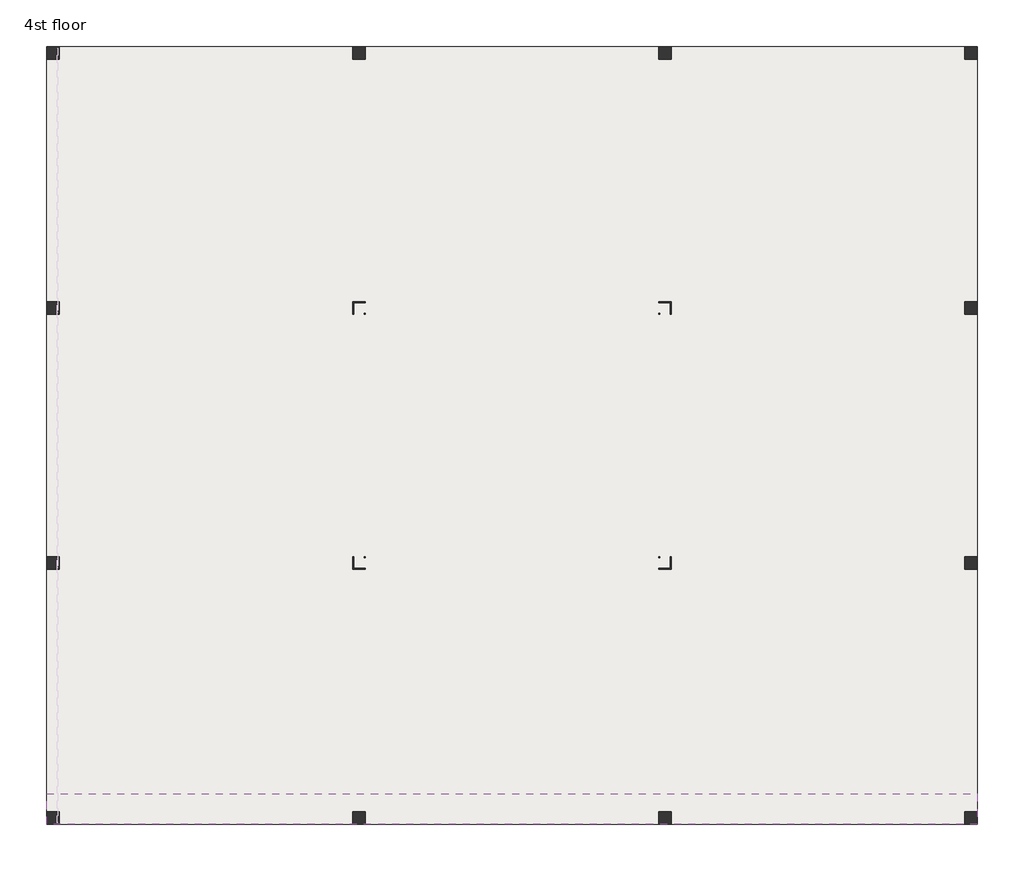
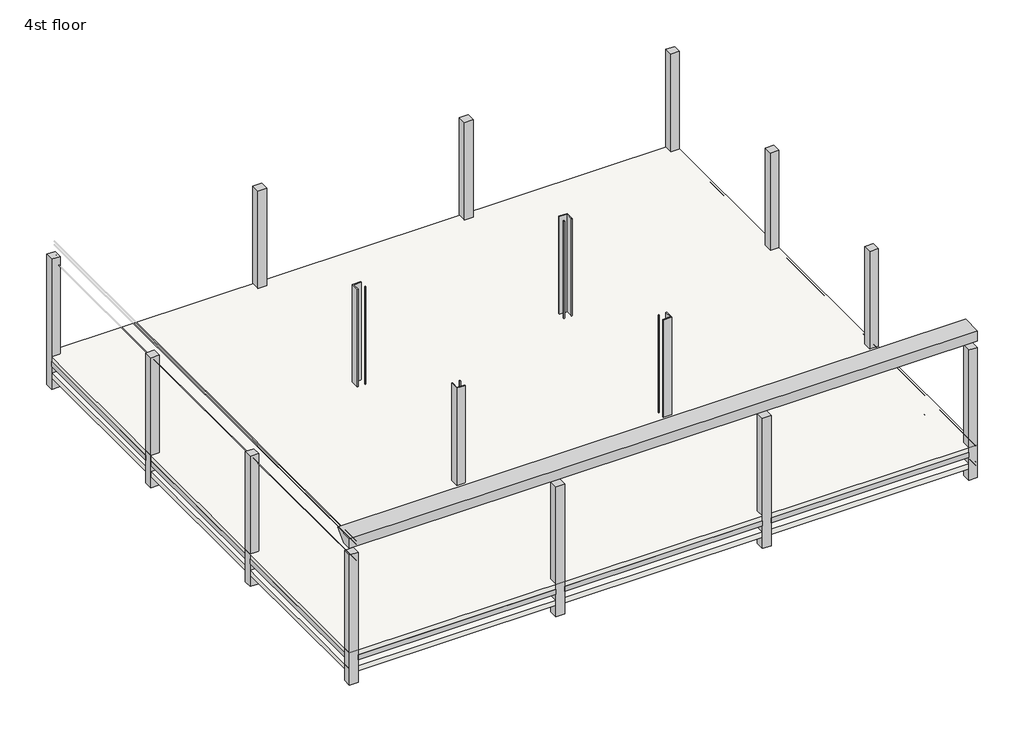
# One storey, part 1 of 2: 24 beams, 16 columns, 2 proxies, 2 slabs.
"""IFC4 building model written with IfcOpenShell, lengths in millimetres."""

import ifcopenshell
import ifcopenshell.guid

model = None  # the IFC model being written
_history = None  # IfcOwnerHistory: only IFC2X3 demands one
_inside = {}  # id of a spatial element -> (the spatial element, [elements in it])
_under = {}  # id of a project, library or spatial element -> (it, [spatial elements below it])
_declared = {}  # id of a project -> (the project, [libraries it declares])
_typed = {}  # id of a type object -> (the type object, [elements of that type])
_made_of = {}  # id of a material, layer set ... -> (it, [elements and type objects made of it])


def new_model(schema):
    """Start an empty IFC model of exactly this schema.

    Asked for "IFC4X3", IfcOpenShell would pick the latest addendum, in which some entities
    have other attributes; the version numbers below select the first issue.
    IFC2X3 requires an IfcOwnerHistory on every rooted entity: one is made here for all.
    """
    global model, _history
    if schema == "IFC4X3":
        model = ifcopenshell.file(schema_version=(4, 3, 0, 0))
    else:
        model = ifcopenshell.file(schema=schema)
    _inside.clear()
    _under.clear()
    _declared.clear()
    _typed.clear()
    _made_of.clear()
    _history = None
    if model.schema == "IFC2X3":
        org = make("IfcOrganization", Name="unknown")
        user = make(
            "IfcPersonAndOrganization",
            ThePerson=make("IfcPerson", FamilyName="unknown"),
            TheOrganization=org,
        )
        app = make(
            "IfcApplication",
            ApplicationDeveloper=org,
            Version="unknown",
            ApplicationFullName="unknown",
            ApplicationIdentifier="unknown",
        )
        _history = make(
            "IfcOwnerHistory",
            OwningUser=user,
            OwningApplication=app,
            ChangeAction="ADDED",
            CreationDate=0,
        )
    return model


def make(cls, **values):
    """One entity of the class cls with the attributes given. An attribute that is None is left unset."""
    return model.create_entity(
        cls, **{name: value for name, value in values.items() if value is not None}
    )


def rooted(cls, **values):
    """An entity with a GlobalId (a new one), such as an element, a storey or a relation."""
    return make(cls, GlobalId=ifcopenshell.guid.new(), OwnerHistory=_history, **values)


def si_unit(unit_type, name, prefix=None):
    """IfcSIUnit, for example si_unit("LENGTHUNIT", "METRE", prefix="MILLI")."""
    return make("IfcSIUnit", UnitType=unit_type, Prefix=prefix, Name=name)


def assignment(units):
    """IfcUnitAssignment: the units of a project."""
    return None if units is None else make("IfcUnitAssignment", Units=units)


def point(xyz):
    """IfcCartesianPoint."""
    return None if xyz is None else make("IfcCartesianPoint", Coordinates=xyz)


def direction(xyz):
    """IfcDirection."""
    return None if xyz is None else make("IfcDirection", DirectionRatios=xyz)


def frame(location, z_axis=None, x_axis=None):
    """IfcAxis2Placement3D, a coordinate frame: its origin and axes. An axis left out is left unset."""
    return make(
        "IfcAxis2Placement3D",
        Location=point(location),
        Axis=direction(z_axis),
        RefDirection=direction(x_axis),
    )


def origin():
    """The frame at (0, 0, 0) with its axes left unset."""
    return frame((0.0, 0.0, 0.0))


def place(relative_to, where):
    """IfcLocalPlacement: puts the frame where relative to a parent placement (None: the world)."""
    return make(
        "IfcLocalPlacement", PlacementRelTo=relative_to, RelativePlacement=where
    )


def context(
    kind, dimensions, precision=None, world=None, true_north=None, identifier=None
):
    """IfcGeometricRepresentationContext, for example the 3D "Model" context."""
    return make(
        "IfcGeometricRepresentationContext",
        ContextIdentifier=identifier,
        ContextType=kind,
        CoordinateSpaceDimension=dimensions,
        Precision=precision,
        WorldCoordinateSystem=world,
        TrueNorth=true_north,
    )


def project(units=None, contexts=None):
    """IfcProject with its units and contexts."""
    return rooted(
        "IfcProject",
        Name="project",
        RepresentationContexts=contexts,
        UnitsInContext=assignment(units),
    )


def spatial(cls, under=None, at=None, **own):
    """A site, building, storey or space (cls), placed at a placement, below another one or the project."""
    s = rooted(cls, ObjectPlacement=at, **own)
    if under is not None:
        _under.setdefault(under.id(), (under, []))[1].append(s)
    return s


def polyline(points):
    """IfcPolyline through the points."""
    return make("IfcPolyline", Points=[point(p) for p in points])


def outline(outer, holes=None, kind="AREA"):
    """IfcArbitraryClosedProfileDef: a profile drawn as a closed curve; with holes, ...WithVoids."""
    if holes is None:
        return make("IfcArbitraryClosedProfileDef", ProfileType=kind, OuterCurve=outer)
    return make(
        "IfcArbitraryProfileDefWithVoids",
        ProfileType=kind,
        OuterCurve=outer,
        InnerCurves=holes,
    )


def extrude(swept, where, along, depth):
    """IfcExtrudedAreaSolid: the profile swept, set in the frame where, extruded along a direction by depth."""
    return make(
        "IfcExtrudedAreaSolid",
        SweptArea=swept,
        Position=where,
        ExtrudedDirection=direction(along),
        Depth=depth,
    )


def faces_of(points, faces, orient=None, outer=None):
    """IfcFace entities. A face is a list of loops; a loop is a list of indices into points, from 0.

    orient and outer hold one flag for each loop. By default every Orientation is true, the
    first loop of a face is its IfcFaceOuterBound and the others are IfcFaceBound.
    """
    made = []
    for i, loops in enumerate(faces):
        bounds = []
        for j, loop in enumerate(loops):
            is_outer = j == 0 if outer is None else outer[i][j]
            bounds.append(
                make(
                    "IfcFaceOuterBound" if is_outer else "IfcFaceBound",
                    Bound=make("IfcPolyLoop", Polygon=[points[k] for k in loop]),
                    Orientation=True if orient is None else orient[i][j],
                )
            )
        made.append(make("IfcFace", Bounds=bounds))
    return made


def faceted_brep(points, faces, orient=None, outer=None, voids=None):
    """IfcFacetedBrep: a solid bounded by flat faces; with voids (closed shells), ...WithVoids."""
    shared = [point(p) for p in points]
    hull = make("IfcClosedShell", CfsFaces=faces_of(shared, faces, orient, outer))
    if voids is None:
        return make("IfcFacetedBrep", Outer=hull)
    return make(
        "IfcFacetedBrepWithVoids",
        Outer=hull,
        Voids=[
            make(cls, CfsFaces=faces_of(shared, fs, o, b)) for cls, fs, o, b in voids
        ],
    )


def shape(context_of_items, identifier, shape_type, items):
    """IfcShapeRepresentation: the items that make up one representation, for example the "Body"."""
    return make(
        "IfcShapeRepresentation",
        ContextOfItems=context_of_items,
        RepresentationIdentifier=identifier,
        RepresentationType=shape_type,
        Items=items,
    )


def made_of(thing, what):
    """Note that an element or type object is made of a material, layer set ...; save() writes the relation."""
    if what is not None:
        _made_of.setdefault(what.id(), (what, []))[1].append(thing)
    return thing


def element(
    cls,
    number,
    at=None,
    inside=None,
    cuts=None,
    type_object=None,
    material=None,
    context=None,
    identifier="Body",
    shape_type=None,
    held_by="IfcProductDefinitionShape",
    body=None,
    shapes=None,
    **own,
):
    """One element of the class cls, such as IfcWall. Its Tag is "e" and its number.

    at: its placement. inside: the storey or other place that contains it. cuts: it is an
    opening in that element (IfcRelVoidsElement). A single representation is given by context,
    identifier, shape_type and body (its items); several are given by shapes. held_by: the class
    of the entity that holds the representations. save() writes the other relations.
    """
    e = rooted(cls, Tag="e%d" % number, ObjectPlacement=at, **own)
    if body is not None:
        shapes = [shape(context, identifier, shape_type, body)]
    if shapes is not None:
        e.Representation = make(held_by, Representations=shapes)
    if inside is not None:
        _inside.setdefault(inside.id(), (inside, []))[1].append(e)
    if cuts is not None:
        rooted(
            "IfcRelVoidsElement", RelatingBuildingElement=cuts, RelatedOpeningElement=e
        )
    if type_object is not None:
        _typed.setdefault(type_object.id(), (type_object, []))[1].append(e)
    return made_of(e, material)


def aggregate(whole, parts):
    """IfcRelAggregates: a whole, such as a stair, and the parts it consists of."""
    return rooted("IfcRelAggregates", RelatingObject=whole, RelatedObjects=parts)


def save(model, path):
    """Write the relations noted so far, then the file.

    IfcRelAggregates (storeys below a building ...), IfcRelContainedInSpatialStructure (elements
    in a storey), IfcRelDefinesByType, IfcRelAssociatesMaterial and IfcRelDeclares: one each for
    every whole, place, type object, material and project.
    """
    for whole, parts in _under.values():
        aggregate(whole, parts)
    for where, things in _inside.values():
        rooted(
            "IfcRelContainedInSpatialStructure",
            RelatedElements=things,
            RelatingStructure=where,
        )
    for kind, things in _typed.values():
        rooted("IfcRelDefinesByType", RelatedObjects=things, RelatingType=kind)
    for what, things in _made_of.values():
        rooted("IfcRelAssociatesMaterial", RelatedObjects=things, RelatingMaterial=what)
    for by, libraries in _declared.values():
        rooted("IfcRelDeclares", RelatingContext=by, RelatedDefinitions=libraries)
    model.write(path)


model = new_model("IFC4")

# Units and contexts
model_context = context("Model", 3, world=origin())
ifc_project = project(units=[si_unit("LENGTHUNIT", "METRE", prefix="MILLI")], contexts=[model_context])

# Site, building, storey
site = spatial("IfcSite", under=ifc_project)
building = spatial("IfcBuilding", under=site)
storey = spatial("IfcBuildingStorey", under=building, Name="4st floor", Elevation=15500.0)

# Beams
placement = place(None, origin())
element("IfcBeam", 1, ObjectType="Concrete-Rectangular Beam : 250 x 300mm", at=placement, inside=storey, context=model_context, shape_type="SweptSolid", body=[
    extrude(outline(polyline([(-8833.7181639, -5693.2383613), (-8833.7181639, -5443.2383613), (-3083.7181639, -5443.2383613), (-3083.7181639, -5693.2383613), (-8833.7181639, -5693.2383613)])), frame((0.0, 0.0, 15200.0), z_axis=(0.0, 0.0, 1.0), x_axis=(1.0, 0.0, 0.0)), (0.0, 0.0, 1.0), 150.0),
])
element("IfcBeam", 2, ObjectType="Concrete-Rectangular Beam : 250 x 300mm", at=placement, inside=storey, context=model_context, shape_type="SweptSolid", body=[
    extrude(outline(polyline([(-2833.7181639, -5693.2383613), (-2833.7181639, -5443.2383613), (2916.2818361, -5443.2383613), (2916.2818361, -5693.2383613), (-2833.7181639, -5693.2383613)])), frame((0.0, 0.0, 15200.0), z_axis=(0.0, 0.0, 1.0), x_axis=(1.0, 0.0, 0.0)), (0.0, 0.0, 1.0), 150.0),
])
element("IfcBeam", 3, ObjectType="Concrete-Rectangular Beam : 250 x 300mm", at=placement, inside=storey, context=model_context, shape_type="SweptSolid", body=[
    extrude(outline(polyline([(3166.2818361, -5693.2383613), (3166.2818361, -5443.2383613), (8916.2818361, -5443.2383613), (8916.2818361, -5693.2383613), (3166.2818361, -5693.2383613)])), frame((0.0, 0.0, 15200.0), z_axis=(0.0, 0.0, 1.0), x_axis=(1.0, 0.0, 0.0)), (0.0, 0.0, 1.0), 150.0),
])
element("IfcBeam", 4, ObjectType="Concrete-Rectangular Beam : 250 x 300mm", at=placement, inside=storey, context=model_context, shape_type="SweptSolid", body=[
    extrude(outline(polyline([(-8833.7181639, -10443.2383613), (-9083.7181639, -10443.2383613), (-9083.7181639, -5693.2383613), (-8833.7181639, -5693.2383613), (-8833.7181639, -10443.2383613)])), frame((0.0, 0.0, 15200.0), z_axis=(0.0, 0.0, 1.0), x_axis=(1.0, 0.0, 0.0)), (0.0, 0.0, 1.0), 150.0),
])
element("IfcBeam", 5, ObjectType="Concrete-Rectangular Beam : 250 x 300mm", at=placement, inside=storey, context=model_context, shape_type="SweptSolid", body=[
    extrude(outline(polyline([(-8833.7181639, -15443.2383613), (-9083.7181639, -15443.2383613), (-9083.7181639, -10693.2383613), (-8833.7181639, -10693.2383613), (-8833.7181639, -15443.2383613)])), frame((0.0, 0.0, 15200.0), z_axis=(0.0, 0.0, 1.0), x_axis=(1.0, 0.0, 0.0)), (0.0, 0.0, 1.0), 150.0),
])
element("IfcBeam", 6, ObjectType="Concrete-Rectangular Beam : 250 x 300mm", at=placement, inside=storey, context=model_context, shape_type="SweptSolid", body=[
    extrude(outline(polyline([(-8833.7181639, -20443.2383613), (-9083.7181639, -20443.2383613), (-9083.7181639, -15693.2383613), (-8833.7181639, -15693.2383613), (-8833.7181639, -20443.2383613)])), frame((0.0, 0.0, 15200.0), z_axis=(0.0, 0.0, 1.0), x_axis=(1.0, 0.0, 0.0)), (0.0, 0.0, 1.0), 150.0),
])
element("IfcBeam", 7, ObjectType="Concrete-Rectangular Beam : 250 x 300mm", at=placement, inside=storey, context=model_context, shape_type="SweptSolid", body=[
    extrude(outline(polyline([(-2833.7181639, -10443.2383613), (-3083.7181639, -10443.2383613), (-3083.7181639, -5693.2383613), (-2833.7181639, -5693.2383613), (-2833.7181639, -10443.2383613)])), frame((0.0, 0.0, 15200.0), z_axis=(0.0, 0.0, 1.0), x_axis=(1.0, 0.0, 0.0)), (0.0, 0.0, 1.0), 150.0),
])
element("IfcBeam", 8, ObjectType="Concrete-Rectangular Beam : 250 x 300mm", at=placement, inside=storey, context=model_context, shape_type="SweptSolid", body=[
    extrude(outline(polyline([(-3083.7181639, -15443.2383613), (-3083.7181639, -10693.2383613), (-3058.7181639, -10693.2383613), (-3058.7181639, -15443.2383613), (-3083.7181639, -15443.2383613)])), frame((0.0, 0.0, 15200.0), z_axis=(0.0, 0.0, 1.0), x_axis=(1.0, 0.0, 0.0)), (0.0, 0.0, 1.0), 150.0),
    extrude(outline(polyline([(-2833.7181639, -10693.2383613), (-2833.7181639, -15443.2383613), (-2858.7181639, -15443.2383613), (-2858.7181639, -10693.2383613), (-2833.7181639, -10693.2383613)])), frame((0.0, 0.0, 15200.0), z_axis=(0.0, 0.0, 1.0), x_axis=(1.0, 0.0, 0.0)), (0.0, 0.0, 1.0), 150.0),
])
element("IfcBeam", 9, ObjectType="Concrete-Rectangular Beam : 250 x 300mm", at=placement, inside=storey, context=model_context, shape_type="SweptSolid", body=[
    extrude(outline(polyline([(-2833.7181639, -20443.2383613), (-3083.7181639, -20443.2383613), (-3083.7181639, -15693.2383613), (-2833.7181639, -15693.2383613), (-2833.7181639, -20443.2383613)])), frame((0.0, 0.0, 15200.0), z_axis=(0.0, 0.0, 1.0), x_axis=(1.0, 0.0, 0.0)), (0.0, 0.0, 1.0), 150.0),
])
element("IfcBeam", 10, ObjectType="Concrete-Rectangular Beam : 250 x 300mm", at=placement, inside=storey, context=model_context, shape_type="SweptSolid", body=[
    extrude(outline(polyline([(3166.2818361, -10443.2383613), (2916.2818361, -10443.2383613), (2916.2818361, -5693.2383613), (3166.2818361, -5693.2383613), (3166.2818361, -10443.2383613)])), frame((0.0, 0.0, 15200.0), z_axis=(0.0, 0.0, 1.0), x_axis=(1.0, 0.0, 0.0)), (0.0, 0.0, 1.0), 150.0),
])
element("IfcBeam", 11, ObjectType="Concrete-Rectangular Beam : 250 x 300mm", at=placement, inside=storey, context=model_context, shape_type="SweptSolid", body=[
    extrude(outline(polyline([(2916.2818361, -15443.2383613), (2916.2818361, -10693.2383613), (2941.2818361, -10693.2383613), (2941.2818361, -15443.2383613), (2916.2818361, -15443.2383613)])), frame((0.0, 0.0, 15200.0), z_axis=(0.0, 0.0, 1.0), x_axis=(1.0, 0.0, 0.0)), (0.0, 0.0, 1.0), 150.0),
    extrude(outline(polyline([(3166.2818361, -10693.2383613), (3166.2818361, -15443.2383613), (3141.2818361, -15443.2383613), (3141.2818361, -10693.2383613), (3166.2818361, -10693.2383613)])), frame((0.0, 0.0, 15200.0), z_axis=(0.0, 0.0, 1.0), x_axis=(1.0, 0.0, 0.0)), (0.0, 0.0, 1.0), 150.0),
])
element("IfcBeam", 12, ObjectType="Concrete-Rectangular Beam : 250 x 300mm", at=placement, inside=storey, context=model_context, shape_type="SweptSolid", body=[
    extrude(outline(polyline([(3166.2818361, -20443.2383613), (2916.2818361, -20443.2383613), (2916.2818361, -15693.2383613), (3166.2818361, -15693.2383613), (3166.2818361, -20443.2383613)])), frame((0.0, 0.0, 15200.0), z_axis=(0.0, 0.0, 1.0), x_axis=(1.0, 0.0, 0.0)), (0.0, 0.0, 1.0), 150.0),
])
element("IfcBeam", 13, ObjectType="Concrete-Rectangular Beam : 250 x 300mm", at=placement, inside=storey, context=model_context, shape_type="SweptSolid", body=[
    extrude(outline(polyline([(9166.2818361, -10443.2383613), (8916.2818361, -10443.2383613), (8916.2818361, -5693.2383613), (9166.2818361, -5693.2383613), (9166.2818361, -10443.2383613)])), frame((0.0, 0.0, 15200.0), z_axis=(0.0, 0.0, 1.0), x_axis=(1.0, 0.0, 0.0)), (0.0, 0.0, 1.0), 150.0),
])
element("IfcBeam", 14, ObjectType="Concrete-Rectangular Beam : 250 x 300mm", at=placement, inside=storey, context=model_context, shape_type="SweptSolid", body=[
    extrude(outline(polyline([(9166.2818361, -15443.2383613), (8916.2818361, -15443.2383613), (8916.2818361, -10693.2383613), (9166.2818361, -10693.2383613), (9166.2818361, -15443.2383613)])), frame((0.0, 0.0, 15200.0), z_axis=(0.0, 0.0, 1.0), x_axis=(1.0, 0.0, 0.0)), (0.0, 0.0, 1.0), 150.0),
])
element("IfcBeam", 15, ObjectType="Concrete-Rectangular Beam : 250 x 300mm", at=placement, inside=storey, context=model_context, shape_type="SweptSolid", body=[
    extrude(outline(polyline([(9166.2818361, -20443.2383613), (8916.2818361, -20443.2383613), (8916.2818361, -15693.2383613), (9166.2818361, -15693.2383613), (9166.2818361, -20443.2383613)])), frame((0.0, 0.0, 15200.0), z_axis=(0.0, 0.0, 1.0), x_axis=(1.0, 0.0, 0.0)), (0.0, 0.0, 1.0), 150.0),
])
element("IfcBeam", 16, ObjectType="Concrete-Rectangular Beam : 250 x 300mm", at=placement, inside=storey, context=model_context, shape_type="SweptSolid", body=[
    extrude(outline(polyline([(-8833.7181639, -20693.2383613), (-8833.7181639, -20443.2383613), (-3083.7181639, -20443.2383613), (-3083.7181639, -20693.2383613), (-8833.7181639, -20693.2383613)])), frame((0.0, 0.0, 15200.0), z_axis=(0.0, 0.0, 1.0), x_axis=(1.0, 0.0, 0.0)), (0.0, 0.0, 1.0), 150.0),
])
element("IfcBeam", 17, ObjectType="Concrete-Rectangular Beam : 250 x 300mm", at=placement, inside=storey, context=model_context, shape_type="SweptSolid", body=[
    extrude(outline(polyline([(-2833.7181639, -20693.2383613), (-2833.7181639, -20443.2383613), (2916.2818361, -20443.2383613), (2916.2818361, -20693.2383613), (-2833.7181639, -20693.2383613)])), frame((0.0, 0.0, 15200.0), z_axis=(0.0, 0.0, 1.0), x_axis=(1.0, 0.0, 0.0)), (0.0, 0.0, 1.0), 150.0),
])
element("IfcBeam", 18, ObjectType="Concrete-Rectangular Beam : 250 x 300mm", at=placement, inside=storey, context=model_context, shape_type="SweptSolid", body=[
    extrude(outline(polyline([(3166.2818361, -20693.2383613), (3166.2818361, -20443.2383613), (8916.2818361, -20443.2383613), (8916.2818361, -20693.2383613), (3166.2818361, -20693.2383613)])), frame((0.0, 0.0, 15200.0), z_axis=(0.0, 0.0, 1.0), x_axis=(1.0, 0.0, 0.0)), (0.0, 0.0, 1.0), 150.0),
])
element("IfcBeam", 19, ObjectType="Concrete-Rectangular Beam : 250 x 300mm", at=placement, inside=storey, context=model_context, shape_type="SweptSolid", body=[
    extrude(outline(polyline([(-8833.7181639, -15693.2383613), (-8833.7181639, -15443.2383613), (-3083.7181639, -15443.2383613), (-3083.7181639, -15693.2383613), (-8833.7181639, -15693.2383613)])), frame((0.0, 0.0, 15200.0), z_axis=(0.0, 0.0, 1.0), x_axis=(1.0, 0.0, 0.0)), (0.0, 0.0, 1.0), 150.0),
])
element("IfcBeam", 20, ObjectType="Concrete-Rectangular Beam : 250 x 300mm", at=placement, inside=storey, context=model_context, shape_type="SweptSolid", body=[
    extrude(outline(polyline([(2916.2818361, -15693.2383613), (-2833.7181639, -15693.2383613), (-2833.7181639, -15668.2383613), (2916.2818361, -15668.2383613), (2916.2818361, -15693.2383613)])), frame((0.0, 0.0, 15200.0), z_axis=(0.0, 0.0, 1.0), x_axis=(1.0, 0.0, 0.0)), (0.0, 0.0, 1.0), 150.0),
    extrude(outline(polyline([(-2833.7181639, -15443.2383613), (2916.2818361, -15443.2383613), (2916.2818361, -15468.2383613), (-2833.7181639, -15468.2383613), (-2833.7181639, -15443.2383613)])), frame((0.0, 0.0, 15200.0), z_axis=(0.0, 0.0, 1.0), x_axis=(1.0, 0.0, 0.0)), (0.0, 0.0, 1.0), 150.0),
])
element("IfcBeam", 21, ObjectType="Concrete-Rectangular Beam : 250 x 300mm", at=placement, inside=storey, context=model_context, shape_type="SweptSolid", body=[
    extrude(outline(polyline([(3166.2818361, -15693.2383613), (3166.2818361, -15443.2383613), (8916.2818361, -15443.2383613), (8916.2818361, -15693.2383613), (3166.2818361, -15693.2383613)])), frame((0.0, 0.0, 15200.0), z_axis=(0.0, 0.0, 1.0), x_axis=(1.0, 0.0, 0.0)), (0.0, 0.0, 1.0), 150.0),
])
element("IfcBeam", 22, ObjectType="Concrete-Rectangular Beam : 250 x 300mm", at=placement, inside=storey, context=model_context, shape_type="SweptSolid", body=[
    extrude(outline(polyline([(-8833.7181639, -10693.2383613), (-8833.7181639, -10443.2383613), (-3083.7181639, -10443.2383613), (-3083.7181639, -10693.2383613), (-8833.7181639, -10693.2383613)])), frame((0.0, 0.0, 15200.0), z_axis=(0.0, 0.0, 1.0), x_axis=(1.0, 0.0, 0.0)), (0.0, 0.0, 1.0), 150.0),
])
element("IfcBeam", 23, ObjectType="Concrete-Rectangular Beam : 250 x 300mm", at=placement, inside=storey, context=model_context, shape_type="SweptSolid", body=[
    extrude(outline(polyline([(2916.2818361, -10693.2383613), (-2833.7181639, -10693.2383613), (-2833.7181639, -10668.2383613), (2916.2818361, -10668.2383613), (2916.2818361, -10693.2383613)])), frame((0.0, 0.0, 15200.0), z_axis=(0.0, 0.0, 1.0), x_axis=(1.0, 0.0, 0.0)), (0.0, 0.0, 1.0), 150.0),
    extrude(outline(polyline([(-2833.7181639, -10443.2383613), (2916.2818361, -10443.2383613), (2916.2818361, -10468.2383613), (-2833.7181639, -10468.2383613), (-2833.7181639, -10443.2383613)])), frame((0.0, 0.0, 15200.0), z_axis=(0.0, 0.0, 1.0), x_axis=(1.0, 0.0, 0.0)), (0.0, 0.0, 1.0), 150.0),
])
element("IfcBeam", 24, ObjectType="Concrete-Rectangular Beam : 250 x 300mm", at=placement, inside=storey, context=model_context, shape_type="SweptSolid", body=[
    extrude(outline(polyline([(3166.2818361, -10693.2383613), (3166.2818361, -10443.2383613), (8916.2818361, -10443.2383613), (8916.2818361, -10693.2383613), (3166.2818361, -10693.2383613)])), frame((0.0, 0.0, 15200.0), z_axis=(0.0, 0.0, 1.0), x_axis=(1.0, 0.0, 0.0)), (0.0, 0.0, 1.0), 150.0),
])

# Proxies
element("IfcBuildingElementProxy", 25, Name="Slab Edge", ObjectType="Slab Edge", at=placement, inside=storey, context=model_context, shape_type="SweptSolid", body=[
    extrude(outline(polyline([(-20693.2383613, 18700.0), (-20693.2383613, 19000.0), (-20093.2383613, 19000.0), (-20393.2383613, 18700.0), (-20693.2383613, 18700.0)])), frame((-9083.7181639, 0.0, 0.0), z_axis=(1.0, 0.0, 0.0), x_axis=(0.0, 1.0, 0.0)), (0.0, 0.0, 1.0), 18250.0),
])
element("IfcBuildingElementProxy", 26, Name="Slab Edge", ObjectType="Slab Edge", at=placement, inside=storey, context=model_context, shape_type="SweptSolid", body=[
    extrude(outline(polyline([(-20693.2383613, 18700.0), (-20693.2383613, 19000.0), (-20093.2383613, 19000.0), (-20393.2383613, 18700.0), (-20693.2383613, 18700.0)])), frame((-9083.7181639, 0.0, 0.0), z_axis=(1.0, 0.0, 0.0), x_axis=(0.0, 1.0, 0.0)), (0.0, 0.0, 1.0), 18250.0),
])

# Columns
element("IfcColumn", 27, ObjectType="Concrete-Rectangular-Column : 250x250 mm", at=placement, inside=storey, context=model_context, shape_type="Brep", body=[
    faceted_brep([(-8833.7181639, -20443.2383613, 18500.0), (-9083.7181639, -20443.2383613, 18500.0), (-9083.7181639, -20693.2383613, 18500.0), (-8833.7181639, -20693.2383613, 18500.0), (-8833.7181639, -20443.2383613, 14500.0), (-8833.7181639, -20693.2383613, 14500.0), (-9083.7181639, -20693.2383613, 14500.0), (-9083.7181639, -20443.2383613, 14500.0), (-8833.7181639, -20443.2383613, 14850.0), (-8833.7181639, -20443.2383613, 14700.0), (-9083.7181639, -20443.2383613, 14700.0), (-9083.7181639, -20443.2383613, 14850.0), (-8833.7181639, -20693.2383613, 14700.0), (-8833.7181639, -20693.2383613, 14850.0)], [[[0, 1, 2, 3]], [[4, 5, 6, 7]], [[1, 0, 8, 9, 4, 7, 10, 11]], [[2, 1, 11, 10, 7, 6]], [[3, 2, 6, 5, 12, 13]], [[0, 3, 13, 12, 5, 4, 9, 8]]]),
])
element("IfcColumn", 28, ObjectType="Concrete-Rectangular-Column : 250x250 mm", at=placement, inside=storey, context=model_context, shape_type="Brep", body=[
    faceted_brep([(-8833.7181639, -15443.2383613, 18500.0), (-9083.7181639, -15443.2383613, 18500.0), (-9083.7181639, -15693.2383613, 18500.0), (-8833.7181639, -15693.2383613, 18500.0), (-8833.7181639, -15443.2383613, 14500.0), (-8833.7181639, -15693.2383613, 14500.0), (-9083.7181639, -15693.2383613, 14500.0), (-9083.7181639, -15443.2383613, 14500.0), (-8833.7181639, -15443.2383613, 14850.0), (-8833.7181639, -15443.2383613, 14700.0), (-9083.7181639, -15443.2383613, 14700.0), (-9083.7181639, -15443.2383613, 14850.0), (-9083.7181639, -15693.2383613, 14700.0), (-9083.7181639, -15693.2383613, 14850.0), (-8833.7181639, -15693.2383613, 14700.0), (-8833.7181639, -15693.2383613, 14850.0)], [[[0, 1, 2, 3]], [[4, 5, 6, 7]], [[1, 0, 8, 9, 4, 7, 10, 11]], [[2, 1, 11, 10, 7, 6, 12, 13]], [[3, 2, 13, 12, 6, 5, 14, 15]], [[0, 3, 15, 14, 5, 4, 9, 8]]]),
])
element("IfcColumn", 29, ObjectType="Concrete-Rectangular-Column : 250x250 mm", at=placement, inside=storey, context=model_context, shape_type="Brep", body=[
    faceted_brep([(-8833.7181639, -10443.2383613, 18500.0), (-9083.7181639, -10443.2383613, 18500.0), (-9083.7181639, -10693.2383613, 18500.0), (-8833.7181639, -10693.2383613, 18500.0), (-8833.7181639, -10443.2383613, 14500.0), (-8833.7181639, -10693.2383613, 14500.0), (-9083.7181639, -10693.2383613, 14500.0), (-9083.7181639, -10443.2383613, 14500.0), (-8833.7181639, -10443.2383613, 14850.0), (-8833.7181639, -10443.2383613, 14700.0), (-9083.7181639, -10443.2383613, 14700.0), (-9083.7181639, -10443.2383613, 14850.0), (-9083.7181639, -10693.2383613, 14700.0), (-9083.7181639, -10693.2383613, 14850.0), (-8833.7181639, -10693.2383613, 14700.0), (-8833.7181639, -10693.2383613, 14850.0)], [[[0, 1, 2, 3]], [[4, 5, 6, 7]], [[1, 0, 8, 9, 4, 7, 10, 11]], [[2, 1, 11, 10, 7, 6, 12, 13]], [[3, 2, 13, 12, 6, 5, 14, 15]], [[0, 3, 15, 14, 5, 4, 9, 8]]]),
])
element("IfcColumn", 30, ObjectType="Concrete-Rectangular-Column : 250x250 mm", at=placement, inside=storey, context=model_context, shape_type="Brep", body=[
    faceted_brep([(-8833.7181639, -5443.2383613, 18500.0), (-9083.7181639, -5443.2383613, 18500.0), (-9083.7181639, -5693.2383613, 18500.0), (-8833.7181639, -5693.2383613, 18500.0), (-8833.7181639, -5443.2383613, 14500.0), (-8833.7181639, -5693.2383613, 14500.0), (-9083.7181639, -5693.2383613, 14500.0), (-9083.7181639, -5443.2383613, 14500.0), (-8833.7181639, -5443.2383613, 14850.0), (-8833.7181639, -5443.2383613, 14700.0), (-9083.7181639, -5693.2383613, 14700.0), (-9083.7181639, -5693.2383613, 14850.0), (-8833.7181639, -5693.2383613, 14700.0), (-8833.7181639, -5693.2383613, 14850.0)], [[[0, 1, 2, 3]], [[4, 5, 6, 7]], [[1, 0, 8, 9, 4, 7]], [[2, 1, 7, 6, 10, 11]], [[3, 2, 11, 10, 6, 5, 12, 13]], [[0, 3, 13, 12, 5, 4, 9, 8]]]),
])
element("IfcColumn", 31, ObjectType="Concrete-Rectangular-Column : 250x250 mm", at=placement, inside=storey, context=model_context, shape_type="Brep", body=[
    faceted_brep([(-2833.7181639, -20443.2383613, 18500.0), (-3083.7181639, -20443.2383613, 18500.0), (-3083.7181639, -20693.2383613, 18500.0), (-2833.7181639, -20693.2383613, 18500.0), (-2833.7181639, -20443.2383613, 14500.0), (-2833.7181639, -20693.2383613, 14500.0), (-3083.7181639, -20693.2383613, 14500.0), (-3083.7181639, -20443.2383613, 14500.0), (-2833.7181639, -20443.2383613, 14850.0), (-2833.7181639, -20443.2383613, 14700.0), (-3083.7181639, -20443.2383613, 14700.0), (-3083.7181639, -20443.2383613, 14850.0), (-3083.7181639, -20693.2383613, 14700.0), (-3083.7181639, -20693.2383613, 14850.0), (-2833.7181639, -20693.2383613, 14700.0), (-2833.7181639, -20693.2383613, 14850.0)], [[[0, 1, 2, 3]], [[4, 5, 6, 7]], [[1, 0, 8, 9, 4, 7, 10, 11]], [[2, 1, 11, 10, 7, 6, 12, 13]], [[3, 2, 13, 12, 6, 5, 14, 15]], [[0, 3, 15, 14, 5, 4, 9, 8]]]),
])
element("IfcColumn", 32, ObjectType="Concrete-Rectangular-Column : 250x250 mm", at=placement, inside=storey, context=model_context, shape_type="Brep", body=[
    faceted_brep([(-2833.7181639, -15468.2383613, 18500.0), (-2833.7181639, -15443.2383613, 18500.0), (-2858.7181639, -15443.2383613, 18500.0), (-2858.7181639, -15468.2383613, 18500.0), (-2833.7181639, -15443.2383613, 14500.0), (-2833.7181639, -15468.2383613, 14500.0), (-2858.7181639, -15468.2383613, 14500.0), (-2858.7181639, -15443.2383613, 14500.0), (-2833.7181639, -15443.2383613, 14850.0), (-2833.7181639, -15443.2383613, 14700.0), (-2858.7181639, -15443.2383613, 14700.0), (-2858.7181639, -15443.2383613, 14850.0), (-2833.7181639, -15468.2383613, 14850.0), (-2833.7181639, -15468.2383613, 14700.0)], [[[0, 1, 2, 3]], [[4, 5, 6, 7]], [[1, 8, 9, 4, 7, 10, 11, 2]], [[4, 9, 8, 1, 0, 12, 13, 5]], [[5, 13, 12, 0, 3, 6]], [[3, 2, 11, 10, 7, 6]]]),
    faceted_brep([(-3083.7181639, -15693.2383613, 18500.0), (-3083.7181639, -15443.2383613, 18500.0), (-3083.7181639, -15443.2383613, 14850.0), (-3083.7181639, -15443.2383613, 14700.0), (-3083.7181639, -15443.2383613, 14500.0), (-3083.7181639, -15693.2383613, 14500.0), (-3083.7181639, -15693.2383613, 14700.0), (-3083.7181639, -15693.2383613, 14850.0), (-2833.7181639, -15693.2383613, 18500.0), (-2833.7181639, -15693.2383613, 14500.0), (-2833.7181639, -15693.2383613, 14700.0), (-2833.7181639, -15693.2383613, 14850.0), (-3058.7181639, -15668.2383613, 14500.0), (-3058.7181639, -15668.2383613, 18500.0), (-2833.7181639, -15668.2383613, 18500.0), (-2833.7181639, -15668.2383613, 14850.0), (-2833.7181639, -15668.2383613, 14700.0), (-2833.7181639, -15668.2383613, 14500.0), (-3058.7181639, -15443.2383613, 14500.0), (-3058.7181639, -15443.2383613, 14700.0), (-3058.7181639, -15443.2383613, 14850.0), (-3058.7181639, -15443.2383613, 18500.0)], [[[0, 1, 2, 3, 4, 5, 6, 7]], [[8, 0, 7, 6, 5, 9, 10, 11]], [[12, 13, 14, 15, 16, 17]], [[13, 12, 18, 19, 20, 21]], [[8, 11, 10, 9, 17, 16, 15, 14]], [[1, 0, 8, 14, 13, 21]], [[9, 5, 4, 18, 12, 17]], [[4, 3, 2, 1, 21, 20, 19, 18]]]),
])
element("IfcColumn", 33, ObjectType="Concrete-Rectangular-Column : 250x250 mm", at=placement, inside=storey, context=model_context, shape_type="Brep", body=[
    faceted_brep([(-2833.7181639, -10443.2383613, 18500.0), (-3083.7181639, -10443.2383613, 18500.0), (-3083.7181639, -10693.2383613, 18500.0), (-3058.7181639, -10693.2383613, 18500.0), (-3058.7181639, -10468.2383613, 18500.0), (-2833.7181639, -10468.2383613, 18500.0), (-3083.7181639, -10693.2383613, 14500.0), (-3083.7181639, -10443.2383613, 14500.0), (-2833.7181639, -10443.2383613, 14500.0), (-2833.7181639, -10468.2383613, 14500.0), (-3058.7181639, -10468.2383613, 14500.0), (-3058.7181639, -10693.2383613, 14500.0), (-2833.7181639, -10443.2383613, 14850.0), (-2833.7181639, -10443.2383613, 14700.0), (-3083.7181639, -10443.2383613, 14700.0), (-3083.7181639, -10443.2383613, 14850.0), (-3083.7181639, -10693.2383613, 14700.0), (-3083.7181639, -10693.2383613, 14850.0), (-3058.7181639, -10693.2383613, 14700.0), (-3058.7181639, -10693.2383613, 14850.0), (-2833.7181639, -10468.2383613, 14850.0), (-2833.7181639, -10468.2383613, 14700.0)], [[[0, 1, 2, 3, 4, 5]], [[6, 7, 8, 9, 10, 11]], [[1, 0, 12, 13, 8, 7, 14, 15]], [[2, 1, 15, 14, 7, 6, 16, 17]], [[2, 17, 16, 6, 11, 18, 19, 3]], [[8, 13, 12, 0, 5, 20, 21, 9]], [[4, 10, 9, 21, 20, 5]], [[10, 4, 3, 19, 18, 11]]]),
    faceted_brep([(-2833.7181639, -10668.2383613, 18500.0), (-2833.7181639, -10668.2383613, 14850.0), (-2833.7181639, -10668.2383613, 14700.0), (-2833.7181639, -10668.2383613, 14500.0), (-2858.7181639, -10668.2383613, 14500.0), (-2858.7181639, -10668.2383613, 18500.0), (-2833.7181639, -10693.2383613, 18500.0), (-2833.7181639, -10693.2383613, 14850.0), (-2833.7181639, -10693.2383613, 14700.0), (-2833.7181639, -10693.2383613, 14500.0), (-2858.7181639, -10693.2383613, 18500.0), (-2858.7181639, -10693.2383613, 14500.0), (-2858.7181639, -10693.2383613, 14700.0), (-2858.7181639, -10693.2383613, 14850.0)], [[[0, 1, 2, 3, 4, 5]], [[6, 7, 8, 9, 3, 2, 1, 0]], [[10, 5, 4, 11, 12, 13]], [[6, 0, 5, 10]], [[3, 9, 11, 4]], [[9, 8, 7, 6, 10, 13, 12, 11]]]),
])
element("IfcColumn", 34, ObjectType="Concrete-Rectangular-Column : 250x250 mm", at=placement, inside=storey, context=model_context, shape_type="Brep", body=[
    faceted_brep([(-2833.7181639, -5443.2383613, 18500.0), (-3083.7181639, -5443.2383613, 18500.0), (-3083.7181639, -5693.2383613, 18500.0), (-2833.7181639, -5693.2383613, 18500.0), (-2833.7181639, -5443.2383613, 14500.0), (-2833.7181639, -5693.2383613, 14500.0), (-3083.7181639, -5693.2383613, 14500.0), (-3083.7181639, -5443.2383613, 14500.0), (-2833.7181639, -5443.2383613, 14850.0), (-2833.7181639, -5443.2383613, 14700.0), (-3083.7181639, -5443.2383613, 14700.0), (-3083.7181639, -5443.2383613, 14850.0), (-3083.7181639, -5693.2383613, 14700.0), (-3083.7181639, -5693.2383613, 14850.0), (-2833.7181639, -5693.2383613, 14700.0), (-2833.7181639, -5693.2383613, 14850.0)], [[[0, 1, 2, 3]], [[4, 5, 6, 7]], [[1, 0, 8, 9, 4, 7, 10, 11]], [[2, 1, 11, 10, 7, 6, 12, 13]], [[3, 2, 13, 12, 6, 5, 14, 15]], [[0, 3, 15, 14, 5, 4, 9, 8]]]),
])
element("IfcColumn", 35, ObjectType="Concrete-Rectangular-Column : 250x250 mm", at=placement, inside=storey, context=model_context, shape_type="Brep", body=[
    faceted_brep([(3166.2818361, -20443.2383613, 18500.0), (2916.2818361, -20443.2383613, 18500.0), (2916.2818361, -20693.2383613, 18500.0), (3166.2818361, -20693.2383613, 18500.0), (3166.2818361, -20443.2383613, 14500.0), (3166.2818361, -20693.2383613, 14500.0), (2916.2818361, -20693.2383613, 14500.0), (2916.2818361, -20443.2383613, 14500.0), (3166.2818361, -20443.2383613, 14850.0), (3166.2818361, -20443.2383613, 14700.0), (2916.2818361, -20443.2383613, 14700.0), (2916.2818361, -20443.2383613, 14850.0), (2916.2818361, -20693.2383613, 14700.0), (2916.2818361, -20693.2383613, 14850.0), (3166.2818361, -20693.2383613, 14700.0), (3166.2818361, -20693.2383613, 14850.0)], [[[0, 1, 2, 3]], [[4, 5, 6, 7]], [[1, 0, 8, 9, 4, 7, 10, 11]], [[2, 1, 11, 10, 7, 6, 12, 13]], [[3, 2, 13, 12, 6, 5, 14, 15]], [[0, 3, 15, 14, 5, 4, 9, 8]]]),
])
element("IfcColumn", 36, ObjectType="Concrete-Rectangular-Column : 250x250 mm", at=placement, inside=storey, context=model_context, shape_type="Brep", body=[
    faceted_brep([(2916.2818361, -15443.2383613, 18500.0), (2916.2818361, -15468.2383613, 18500.0), (2941.2818361, -15468.2383613, 18500.0), (2941.2818361, -15443.2383613, 18500.0), (2916.2818361, -15468.2383613, 14500.0), (2916.2818361, -15443.2383613, 14500.0), (2941.2818361, -15443.2383613, 14500.0), (2941.2818361, -15468.2383613, 14500.0), (2916.2818361, -15443.2383613, 14850.0), (2916.2818361, -15443.2383613, 14700.0), (2916.2818361, -15468.2383613, 14700.0), (2916.2818361, -15468.2383613, 14850.0), (2941.2818361, -15443.2383613, 14700.0), (2941.2818361, -15443.2383613, 14850.0)], [[[0, 1, 2, 3]], [[4, 5, 6, 7]], [[0, 8, 9, 5, 4, 10, 11, 1]], [[1, 11, 10, 4, 7, 2]], [[3, 2, 7, 6, 12, 13]], [[5, 9, 8, 0, 3, 13, 12, 6]]]),
    faceted_brep([(3166.2818361, -15443.2383613, 18500.0), (3166.2818361, -15443.2383613, 14850.0), (3166.2818361, -15443.2383613, 14700.0), (3166.2818361, -15443.2383613, 14500.0), (3141.2818361, -15443.2383613, 14500.0), (3141.2818361, -15443.2383613, 14700.0), (3141.2818361, -15443.2383613, 14850.0), (3141.2818361, -15443.2383613, 18500.0), (3166.2818361, -15693.2383613, 18500.0), (2916.2818361, -15693.2383613, 18500.0), (2916.2818361, -15693.2383613, 14850.0), (2916.2818361, -15693.2383613, 14700.0), (2916.2818361, -15693.2383613, 14500.0), (3166.2818361, -15693.2383613, 14500.0), (3166.2818361, -15693.2383613, 14700.0), (3166.2818361, -15693.2383613, 14850.0), (3141.2818361, -15668.2383613, 18500.0), (3141.2818361, -15668.2383613, 14500.0), (2916.2818361, -15668.2383613, 14500.0), (2916.2818361, -15668.2383613, 14700.0), (2916.2818361, -15668.2383613, 14850.0), (2916.2818361, -15668.2383613, 18500.0)], [[[0, 1, 2, 3, 4, 5, 6, 7]], [[8, 9, 10, 11, 12, 13, 14, 15]], [[0, 8, 15, 14, 13, 3, 2, 1]], [[16, 17, 18, 19, 20, 21]], [[17, 16, 7, 6, 5, 4]], [[12, 11, 10, 9, 21, 20, 19, 18]], [[9, 8, 0, 7, 16, 21]], [[3, 13, 12, 18, 17, 4]]]),
])
element("IfcColumn", 37, ObjectType="Concrete-Rectangular-Column : 250x250 mm", at=placement, inside=storey, context=model_context, shape_type="Brep", body=[
    faceted_brep([(3166.2818361, -10443.2383613, 18500.0), (2916.2818361, -10443.2383613, 18500.0), (2916.2818361, -10468.2383613, 18500.0), (3141.2818361, -10468.2383613, 18500.0), (3141.2818361, -10693.2383613, 18500.0), (3166.2818361, -10693.2383613, 18500.0), (3166.2818361, -10443.2383613, 14850.0), (3166.2818361, -10443.2383613, 14700.0), (3166.2818361, -10443.2383613, 14500.0), (2916.2818361, -10443.2383613, 14500.0), (2916.2818361, -10443.2383613, 14700.0), (2916.2818361, -10443.2383613, 14850.0), (2916.2818361, -10468.2383613, 14500.0), (2916.2818361, -10468.2383613, 14700.0), (2916.2818361, -10468.2383613, 14850.0), (3166.2818361, -10693.2383613, 14850.0), (3166.2818361, -10693.2383613, 14700.0), (3166.2818361, -10693.2383613, 14500.0), (3141.2818361, -10468.2383613, 14500.0), (3141.2818361, -10693.2383613, 14500.0), (3141.2818361, -10693.2383613, 14700.0), (3141.2818361, -10693.2383613, 14850.0)], [[[0, 1, 2, 3, 4, 5]], [[1, 0, 6, 7, 8, 9, 10, 11]], [[1, 11, 10, 9, 12, 13, 14, 2]], [[0, 5, 15, 16, 17, 8, 7, 6]], [[18, 3, 2, 14, 13, 12]], [[3, 18, 19, 20, 21, 4]], [[8, 17, 19, 18, 12, 9]], [[17, 16, 15, 5, 4, 21, 20, 19]]]),
    faceted_brep([(2916.2818361, -10693.2383613, 14500.0), (2916.2818361, -10668.2383613, 14500.0), (2941.2818361, -10668.2383613, 14500.0), (2941.2818361, -10693.2383613, 14500.0), (2916.2818361, -10693.2383613, 18500.0), (2916.2818361, -10693.2383613, 14850.0), (2916.2818361, -10693.2383613, 14700.0), (2941.2818361, -10693.2383613, 14700.0), (2941.2818361, -10693.2383613, 14850.0), (2941.2818361, -10693.2383613, 18500.0), (2916.2818361, -10668.2383613, 14700.0), (2916.2818361, -10668.2383613, 14850.0), (2916.2818361, -10668.2383613, 18500.0), (2941.2818361, -10668.2383613, 18500.0)], [[[0, 1, 2, 3]], [[4, 5, 6, 0, 3, 7, 8, 9]], [[1, 10, 11, 12, 13, 2]], [[0, 6, 5, 4, 12, 11, 10, 1]], [[13, 9, 8, 7, 3, 2]], [[12, 4, 9, 13]]]),
])
element("IfcColumn", 38, ObjectType="Concrete-Rectangular-Column : 250x250 mm", at=placement, inside=storey, context=model_context, shape_type="Brep", body=[
    faceted_brep([(3166.2818361, -5443.2383613, 18500.0), (2916.2818361, -5443.2383613, 18500.0), (2916.2818361, -5693.2383613, 18500.0), (3166.2818361, -5693.2383613, 18500.0), (3166.2818361, -5443.2383613, 14500.0), (3166.2818361, -5693.2383613, 14500.0), (2916.2818361, -5693.2383613, 14500.0), (2916.2818361, -5443.2383613, 14500.0), (3166.2818361, -5443.2383613, 14850.0), (3166.2818361, -5443.2383613, 14700.0), (2916.2818361, -5443.2383613, 14700.0), (2916.2818361, -5443.2383613, 14850.0), (2916.2818361, -5693.2383613, 14700.0), (2916.2818361, -5693.2383613, 14850.0), (3166.2818361, -5693.2383613, 14700.0), (3166.2818361, -5693.2383613, 14850.0)], [[[0, 1, 2, 3]], [[4, 5, 6, 7]], [[1, 0, 8, 9, 4, 7, 10, 11]], [[2, 1, 11, 10, 7, 6, 12, 13]], [[3, 2, 13, 12, 6, 5, 14, 15]], [[0, 3, 15, 14, 5, 4, 9, 8]]]),
])
element("IfcColumn", 39, ObjectType="Concrete-Rectangular-Column : 250x250 mm", at=placement, inside=storey, context=model_context, shape_type="Brep", body=[
    faceted_brep([(9166.2818361, -20443.2383613, 18500.0), (8916.2818361, -20443.2383613, 18500.0), (8916.2818361, -20693.2383613, 18500.0), (9166.2818361, -20693.2383613, 18500.0), (9166.2818361, -20443.2383613, 14500.0), (9166.2818361, -20693.2383613, 14500.0), (8916.2818361, -20693.2383613, 14500.0), (8916.2818361, -20443.2383613, 14500.0), (9166.2818361, -20443.2383613, 14850.0), (9166.2818361, -20443.2383613, 14700.0), (8916.2818361, -20443.2383613, 14700.0), (8916.2818361, -20443.2383613, 14850.0), (8916.2818361, -20693.2383613, 14700.0), (8916.2818361, -20693.2383613, 14850.0)], [[[0, 1, 2, 3]], [[4, 5, 6, 7]], [[1, 0, 8, 9, 4, 7, 10, 11]], [[2, 1, 11, 10, 7, 6, 12, 13]], [[3, 2, 13, 12, 6, 5]], [[0, 3, 5, 4, 9, 8]]]),
])
element("IfcColumn", 40, ObjectType="Concrete-Rectangular-Column : 250x250 mm", at=placement, inside=storey, context=model_context, shape_type="Brep", body=[
    faceted_brep([(9166.2818361, -15443.2383613, 18500.0), (8916.2818361, -15443.2383613, 18500.0), (8916.2818361, -15693.2383613, 18500.0), (9166.2818361, -15693.2383613, 18500.0), (9166.2818361, -15443.2383613, 14500.0), (9166.2818361, -15693.2383613, 14500.0), (8916.2818361, -15693.2383613, 14500.0), (8916.2818361, -15443.2383613, 14500.0), (9166.2818361, -15443.2383613, 14850.0), (9166.2818361, -15443.2383613, 14700.0), (8916.2818361, -15443.2383613, 14700.0), (8916.2818361, -15443.2383613, 14850.0), (8916.2818361, -15693.2383613, 14700.0), (8916.2818361, -15693.2383613, 14850.0), (9166.2818361, -15693.2383613, 14700.0), (9166.2818361, -15693.2383613, 14850.0)], [[[0, 1, 2, 3]], [[4, 5, 6, 7]], [[1, 0, 8, 9, 4, 7, 10, 11]], [[2, 1, 11, 10, 7, 6, 12, 13]], [[3, 2, 13, 12, 6, 5, 14, 15]], [[0, 3, 15, 14, 5, 4, 9, 8]]]),
])
element("IfcColumn", 41, ObjectType="Concrete-Rectangular-Column : 250x250 mm", at=placement, inside=storey, context=model_context, shape_type="Brep", body=[
    faceted_brep([(9166.2818361, -10443.2383613, 18500.0), (8916.2818361, -10443.2383613, 18500.0), (8916.2818361, -10693.2383613, 18500.0), (9166.2818361, -10693.2383613, 18500.0), (9166.2818361, -10443.2383613, 14500.0), (9166.2818361, -10693.2383613, 14500.0), (8916.2818361, -10693.2383613, 14500.0), (8916.2818361, -10443.2383613, 14500.0), (9166.2818361, -10443.2383613, 14850.0), (9166.2818361, -10443.2383613, 14700.0), (8916.2818361, -10443.2383613, 14700.0), (8916.2818361, -10443.2383613, 14850.0), (8916.2818361, -10693.2383613, 14700.0), (8916.2818361, -10693.2383613, 14850.0), (9166.2818361, -10693.2383613, 14700.0), (9166.2818361, -10693.2383613, 14850.0)], [[[0, 1, 2, 3]], [[4, 5, 6, 7]], [[1, 0, 8, 9, 4, 7, 10, 11]], [[2, 1, 11, 10, 7, 6, 12, 13]], [[3, 2, 13, 12, 6, 5, 14, 15]], [[0, 3, 15, 14, 5, 4, 9, 8]]]),
])
element("IfcColumn", 42, ObjectType="Concrete-Rectangular-Column : 250x250 mm", at=placement, inside=storey, context=model_context, shape_type="Brep", body=[
    faceted_brep([(9166.2818361, -5443.2383613, 18500.0), (8916.2818361, -5443.2383613, 18500.0), (8916.2818361, -5693.2383613, 18500.0), (9166.2818361, -5693.2383613, 18500.0), (9166.2818361, -5443.2383613, 14500.0), (9166.2818361, -5693.2383613, 14500.0), (8916.2818361, -5693.2383613, 14500.0), (8916.2818361, -5443.2383613, 14500.0), (8916.2818361, -5443.2383613, 14700.0), (8916.2818361, -5443.2383613, 14850.0), (8916.2818361, -5693.2383613, 14700.0), (8916.2818361, -5693.2383613, 14850.0), (9166.2818361, -5693.2383613, 14700.0), (9166.2818361, -5693.2383613, 14850.0)], [[[0, 1, 2, 3]], [[4, 5, 6, 7]], [[1, 0, 4, 7, 8, 9]], [[2, 1, 9, 8, 7, 6, 10, 11]], [[3, 2, 11, 10, 6, 5, 12, 13]], [[0, 3, 13, 12, 5, 4]]]),
])

# Slabs
element("IfcSlab", 43, ObjectType="150mm Foundation Slab", at=placement, inside=storey, context=model_context, shape_type="Brep", body=[
    faceted_brep([(-9083.7181639, -5443.2383613, 14850.0), (-8833.7181639, -5443.2383613, 14850.0), (-3083.7181639, -5443.2383613, 14850.0), (-2833.7181639, -5443.2383613, 14850.0), (2916.2818361, -5443.2383613, 14850.0), (3166.2818361, -5443.2383613, 14850.0), (8916.2818361, -5443.2383613, 14850.0), (9166.2818361, -5443.2383613, 14850.0), (9166.2818361, -5693.2383613, 14850.0), (9166.2818361, -10443.2383613, 14850.0), (9166.2818361, -10693.2383613, 14850.0), (9166.2818361, -15443.2383613, 14850.0), (9166.2818361, -15693.2383613, 14850.0), (9166.2818361, -20443.2383613, 14850.0), (9166.2818361, -20693.2383613, 14850.0), (8916.2818361, -20693.2383613, 14850.0), (3166.2818361, -20693.2383613, 14850.0), (2916.2818361, -20693.2383613, 14850.0), (-2833.7181639, -20693.2383613, 14850.0), (-3083.7181639, -20693.2383613, 14850.0), (-8833.7181639, -20693.2383613, 14850.0), (-9083.7181639, -20693.2383613, 14850.0), (-9083.7181639, -20443.2383613, 14850.0), (-9083.7181639, -15693.2383613, 14850.0), (-9083.7181639, -15443.2383613, 14850.0), (-9083.7181639, -10693.2383613, 14850.0), (-9083.7181639, -10443.2383613, 14850.0), (-9083.7181639, -5693.2383613, 14850.0), (-9083.7181639, -5443.2383613, 15000.0), (-9083.7181639, -20693.2383613, 15000.0), (9166.2818361, -20693.2383613, 15000.0), (9166.2818361, -5443.2383613, 15000.0)], [[[0, 1, 2, 3, 4, 5, 6, 7, 8, 9, 10, 11, 12, 13, 14, 15, 16, 17, 18, 19, 20, 21, 22, 23, 24, 25, 26, 27]], [[28, 29, 30, 31]], [[7, 6, 5, 4, 3, 2, 1, 0, 28, 31]], [[14, 13, 12, 11, 10, 9, 8, 7, 31, 30]], [[21, 20, 19, 18, 17, 16, 15, 14, 30, 29]], [[0, 27, 26, 25, 24, 23, 22, 21, 29, 28]]]),
])
element("IfcSlab", 44, ObjectType="150mm Foundation Slab", at=placement, inside=storey, context=model_context, shape_type="Brep", body=[
    faceted_brep([(-9083.7181639, -5443.2383613, 15350.0), (-8833.7181639, -5443.2383613, 15350.0), (-3083.7181639, -5443.2383613, 15350.0), (-2833.7181639, -5443.2383613, 15350.0), (2916.2818361, -5443.2383613, 15350.0), (3166.2818361, -5443.2383613, 15350.0), (8916.2818361, -5443.2383613, 15350.0), (9166.2818361, -5443.2383613, 15350.0), (9166.2818361, -5693.2383613, 15350.0), (9166.2818361, -10443.2383613, 15350.0), (9166.2818361, -10693.2383613, 15350.0), (9166.2818361, -15443.2383613, 15350.0), (9166.2818361, -15693.2383613, 15350.0), (9166.2818361, -20443.2383613, 15350.0), (9166.2818361, -20693.2383613, 15350.0), (8916.2818361, -20693.2383613, 15350.0), (3166.2818361, -20693.2383613, 15350.0), (2916.2818361, -20693.2383613, 15350.0), (-2833.7181639, -20693.2383613, 15350.0), (-3083.7181639, -20693.2383613, 15350.0), (-8833.7181639, -20693.2383613, 15350.0), (-9083.7181639, -20693.2383613, 15350.0), (-9083.7181639, -20443.2383613, 15350.0), (-9083.7181639, -15693.2383613, 15350.0), (-9083.7181639, -15443.2383613, 15350.0), (-9083.7181639, -10693.2383613, 15350.0), (-9083.7181639, -10443.2383613, 15350.0), (-9083.7181639, -5693.2383613, 15350.0), (-9083.7181639, -5443.2383613, 15500.0), (-9083.7181639, -20693.2383613, 15500.0), (9166.2818361, -20693.2383613, 15500.0), (9166.2818361, -5443.2383613, 15500.0)], [[[0, 1, 2, 3, 4, 5, 6, 7, 8, 9, 10, 11, 12, 13, 14, 15, 16, 17, 18, 19, 20, 21, 22, 23, 24, 25, 26, 27]], [[28, 29, 30, 31]], [[7, 6, 5, 4, 3, 2, 1, 0, 28, 31]], [[14, 13, 12, 11, 10, 9, 8, 7, 31, 30]], [[21, 20, 19, 18, 17, 16, 15, 14, 30, 29]], [[0, 27, 26, 25, 24, 23, 22, 21, 29, 28]]]),
])

save(model, "model.ifc")

# Revit data of these elements
# Type "Concrete-Rectangular Beam : 250 x 300mm"
#   Length [instance default] = 1524 mm
#   b = 250 mm
#   h = 300 mm
#   Structural Material [instance default] = Concrete, Cast-in-Place gray
#   Assembly Code = ""
# Type "Concrete-Rectangular-Column : 250x250 mm"
#   b = 250 mm
#   h = 250 mm
#   Structural Material [instance default] = Concrete, Cast-in-Place gray
# Type "150mm Foundation Slab"
#   Layers, outside or top first: 150 mm "Concrete, Cast-in-Place gray" (function 1)
# Elements 1, 2, 3, 4, 5, 6, 7, 8, 9, 10, 11, 12, 13, 14, 15, 16, 17, 18, 19, 20, 21, 22, 23, 24 (IfcBeam, "Concrete-Rectangular Beam : 250 x 300mm")
#   Structural Material = Concrete, Cast-in-Place gray
#   Phase Created = New Construction
#   Materials on its faces: "Concrete, Cast-in-Place gray"
# Elements 25, 26 (IfcBuildingElementProxy, "Slab Edge")
#   Phase Created = New Construction
#   Materials on its faces: "Default Floor"
# Elements 27, 28, 29, 30, 31, 32, 33, 34, 35, 36, 37, 38, 39, 40, 41, 42 (IfcColumn, "Concrete-Rectangular-Column : 250x250 mm")
#   Structural Material = Concrete, Cast-in-Place gray
#   Phase Created = New Construction
#   Materials on its faces: "Concrete, Cast-in-Place gray"
# Element 43 (IfcSlab, "150mm Foundation Slab")
#   built-in parameter 1001955 = 3.14159 (stored number, unit not read)
#   Height Offset From Level = -500 mm
#   built-in parameter 1001954 = 1
#   Phase Created = New Construction
#   Materials on its faces: "Concrete, Cast-in-Place gray"
# Element 44 (IfcSlab, "150mm Foundation Slab")
#   built-in parameter 1001955 = 3.14159 (stored number, unit not read)
#   Height Offset From Level = 0 mm
#   built-in parameter 1001954 = 1
#   Phase Created = New Construction
#   Materials on its faces: "Concrete, Cast-in-Place gray"
# Materials
#   "Concrete, Cast-in-Place gray": class "Concrete", colour RGB 192 192 192, transparency 0, Description = "Cast-in-place concrete", Cost = 0
#   "Default Floor": class "Miscellaneous", colour RGB 127 127 127, transparency 0, Cost = 0
